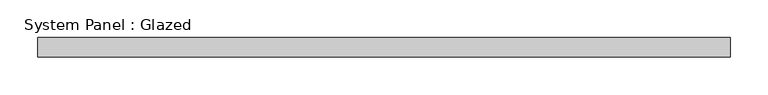
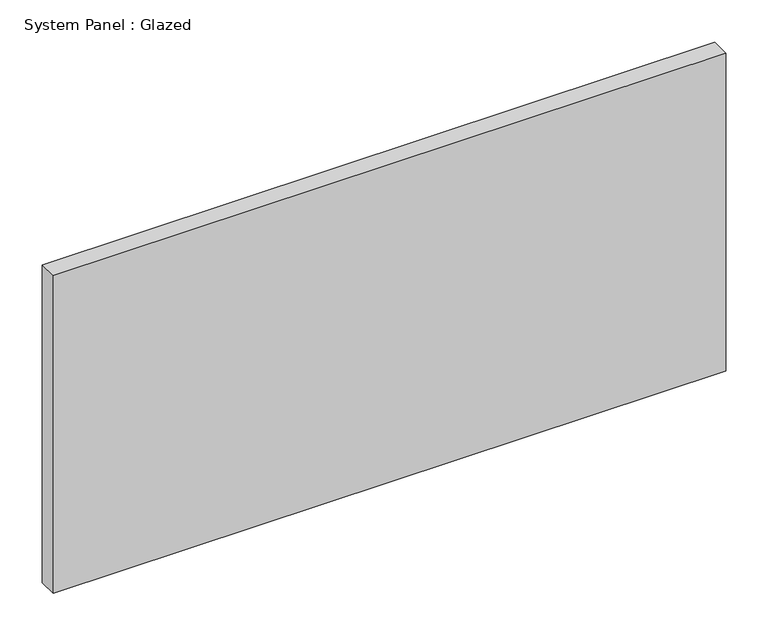
"""IFC4 building model written with IfcOpenShell, lengths in millimetres: plate geometry, System Panel : Glazed."""

from ifc_helpers import new_model, si_unit, origin, origin_with_axes, place, context, project, spatial, polyline, outline, extrude, source, transform, mapped, element, save


def system_panel_glazed_8c5bd8b1(model_context):
    return source(origin(), model_context, "Body", "SweptSolid", [
        extrude(outline(polyline([(457.2, 19.05), (-457.2, 19.05), (-457.2, 44.45), (457.2, 44.45), (457.2, 19.05)])), origin_with_axes(), (0.0, 0.0, 1.0), 457.2),
    ])


if __name__ == "__main__":
    model = new_model("IFC4")
    model_context = context("Model", 3, world=origin())
    ifc_project = project(units=[si_unit("LENGTHUNIT", "METRE", prefix="MILLI")], contexts=[model_context])
    site = spatial("IfcSite", under=ifc_project)
    building = spatial("IfcBuilding", under=site)
    placement = place(None, origin())
    system_panel_glazed_shape = system_panel_glazed_8c5bd8b1(model_context)
    element("IfcPlate", 1, ObjectType="System Panel : Glazed", at=placement, inside=building, context=model_context, shape_type="MappedRepresentation", body=[
        mapped(system_panel_glazed_shape, transform((0.0, 0.0, 0.0), x_axis=(1.0, 0.0, 0.0), y_axis=(0.0, 1.0, 0.0), z_axis=(0.0, 0.0, 1.0))),
    ])
    save(model, "model.ifc")

# Revit data of these elements
# Element 1 (IfcPlate, "System Panel : Glazed")
#   Materials on its faces: "Glass"
# Materials
#   "Glass": class "Glass", colour RGB 0 128 192, transparency 0.75
